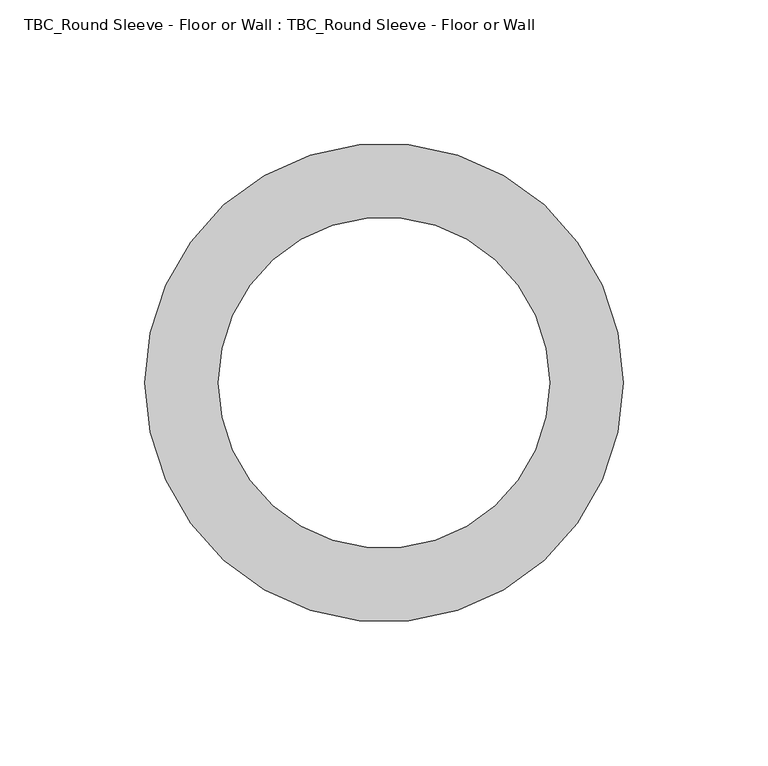
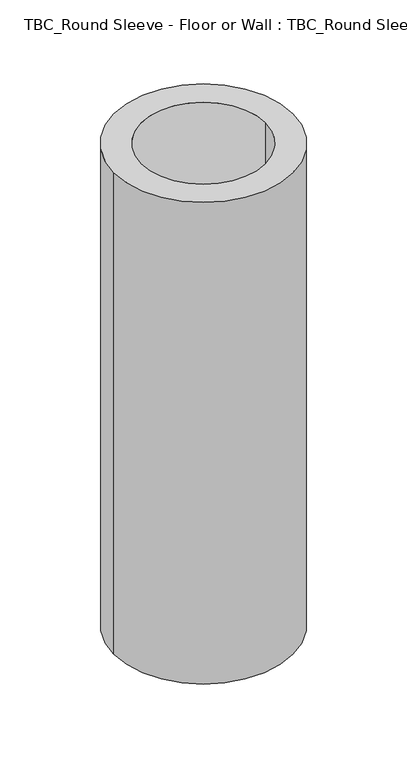
"""IFC4 building model written with IfcOpenShell, lengths in millimetres: proxy geometry, TBC_Round Sleeve - Floor or Wall : TBC_Round Sleeve - Floor or Wall."""

from ifc_helpers import new_model, si_unit, point, frame, origin, origin_2d, place, context, project, spatial, circle_curve, trimmed, segment, composite_curve, outline, extrude, source, transform, mapped, element, save


def tbc_round_sleeve_floor_or_wall_tbc_round_sleeve_floor_or_fd2a9858(model_context):
    return source(origin(), model_context, "Body", "SweptSolid", [
        extrude(outline(composite_curve([segment(trimmed(circle_curve(origin_2d(), 82.55), [point((-82.55, 0.0))], [point((82.55, 0.0))], False, "CARTESIAN"), True, "CONTINUOUS"), segment(trimmed(circle_curve(origin_2d(), 82.55), [point((82.55, 0.0))], [point((-82.55, 0.0))], False, "CARTESIAN"), True, "CONTINUOUS")], self_intersect=False), holes=[composite_curve([segment(trimmed(circle_curve(origin_2d(), 57.15), [point((-57.15, 0.0))], [point((57.15, 0.0))], True, "CARTESIAN"), True, "CONTINUOUS"), segment(trimmed(circle_curve(origin_2d(), 57.15), [point((57.15, 0.0))], [point((-57.15, 0.0))], True, "CARTESIAN"), True, "CONTINUOUS")], self_intersect=False)]), frame((0.0, 0.0, -469.9), z_axis=(0.0, 0.0, 1.0), x_axis=(1.0, 0.0, 0.0)), (0.0, 0.0, 1.0), 469.9),
    ])


if __name__ == "__main__":
    model = new_model("IFC4")
    model_context = context("Model", 3, world=origin())
    ifc_project = project(units=[si_unit("LENGTHUNIT", "METRE", prefix="MILLI")], contexts=[model_context])
    site = spatial("IfcSite", under=ifc_project)
    building = spatial("IfcBuilding", under=site)
    placement = place(None, origin())
    tbc_round_sleeve_floor_or_wall_tbc_round_sleeve_floor_or_shape = tbc_round_sleeve_floor_or_wall_tbc_round_sleeve_floor_or_fd2a9858(model_context)
    element("IfcBuildingElementProxy", 1, Name="TBC_Round Sleeve - Floor or Wall : TBC_Round Sleeve - Floor or Wall", ObjectType="TBC_Round Sleeve - Floor or Wall : TBC_Round Sleeve - Floor or Wall", at=placement, inside=building, context=model_context, shape_type="MappedRepresentation", body=[
        mapped(tbc_round_sleeve_floor_or_wall_tbc_round_sleeve_floor_or_shape, transform((0.0, 0.0, 0.0), x_axis=(1.0, 0.0, 0.0), y_axis=(0.0, 1.0, 0.0), z_axis=(0.0, 0.0, 1.0))),
    ])
    save(model, "model.ifc")

# Revit data of these elements
# Type "TBC_Round Sleeve - Floor or Wall : TBC_Round Sleeve - Floor or Wall"
#   Tag Dimension [instance default] = ""
#   MEP Type [instance default] = ""
#   MEP Element [instance default] = ""
#   MEP Category [instance default] = ""
#   Host Element Type [instance default] = ""
#   Host Element Id [instance default] = ""
#   Host Element Category [instance default] = ""
#   Control Line Y [instance default] = ""
#   Control Line X [instance default] = ""
#   Sleeve Radius [instance default] = 1' - 0"
#   Sleeve Edge [instance default] = 1' - 2"
#   Sleeve Depth [instance default] = 3' - 0"
#   Distance Y [instance default] = 0' - 0"
#   Distance X [instance default] = 0' - 0"
#   Default Elevation = 0
# Element 1 (IfcBuildingElementProxy, "TBC_Round Sleeve - Floor or Wall : TBC_Round Sleeve - Floor or Wall")
#   MEP Element = "895468"
#   MEP Category = "Pipe"
#   Host Element Type = "Roof Plank-Sleeves"
#   Host Element Id = "1525183"
#   Host Element Category = "Floors"
#   Control Line Y = "Y4"
#   Control Line X = "X"
#   Sleeve Radius = 0' - 4 1/2"
#   Sleeve Edge = 0' - 6 1/2"
#   Sleeve Depth = 1' - 6 1/2"
#   Distance Y = 0' - 10.92"
#   Distance X = 5' - 4.8"
